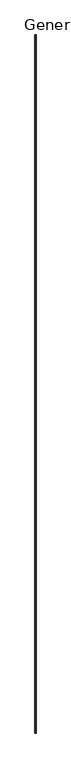
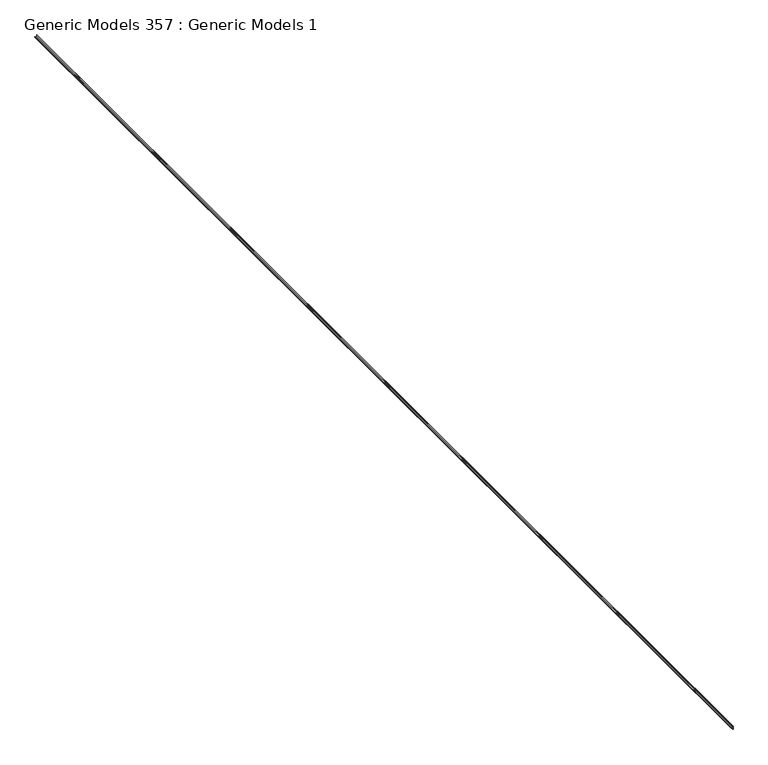
"""IFC4 building model written with IfcOpenShell, lengths in millimetres: proxy geometry, Generic Models 357 : Generic Models 1."""

from ifc_helpers import new_model, si_unit, frame, origin, place, context, project, spatial, polyline, outline, extrude, source, transform, mapped, element, save


def generic_models_357_generic_models_1_35770bf2(model_context):
    return source(origin(), model_context, "Body", "SweptSolid", [
        extrude(outline(polyline([(126669.546, -8716.3018945), (126708.916, -8716.3018945), (126708.916, -8717.5718945), (126689.866, -8717.5718945), (126689.866, -8737.2568945), (126693.3458, -8737.2568945), (126693.3458, -8738.5268945), (126688.596, -8738.5268945), (126688.596, -8717.5718945), (126669.546, -8717.5718945), (126669.546, -8716.3018945)])), frame((0.0, -7068.1230338, 0.0), z_axis=(0.0, 1.0, 0.0), x_axis=(0.0, 0.0, 1.0)), (0.0, 0.0, 1.0), 14122.4),
    ])


if __name__ == "__main__":
    model = new_model("IFC4")
    model_context = context("Model", 3, world=origin())
    ifc_project = project(units=[si_unit("LENGTHUNIT", "METRE", prefix="MILLI")], contexts=[model_context])
    site = spatial("IfcSite", under=ifc_project)
    building = spatial("IfcBuilding", under=site)
    placement = place(None, origin())
    generic_models_357_generic_models_1_shape = generic_models_357_generic_models_1_35770bf2(model_context)
    element("IfcBuildingElementProxy", 1, Name="Generic Models 357 : Generic Models 1", ObjectType="Generic Models 357 : Generic Models 1", at=placement, inside=building, context=model_context, shape_type="MappedRepresentation", body=[
        mapped(generic_models_357_generic_models_1_shape, transform((0.0, 0.0, 0.0), x_axis=(1.0, 0.0, 0.0), y_axis=(0.0, 1.0, 0.0), z_axis=(0.0, 0.0, 1.0))),
    ])
    save(model, "model.ifc")

# Revit data of these elements
# Element 1 (IfcBuildingElementProxy, "Generic Models 357 : Generic Models 1")
#   Materials on its faces: "_ 16 GA. COPPER VENTED T REVEAL BEAD (CONT. AROUND PERIMETER OF BEAM)"
# Materials
#   "_ 16 GA. COPPER VENTED T REVEAL BEAD (CONT. AROUND PERIMETER OF BEAM)": class "Generic", colour RGB 253 192 103, transparency 0, Cost = 0
